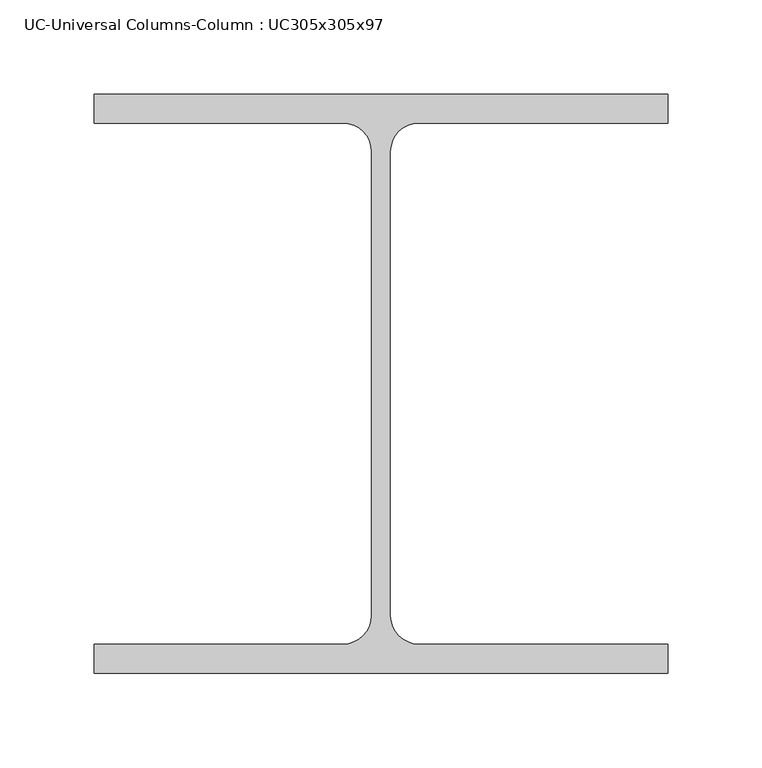
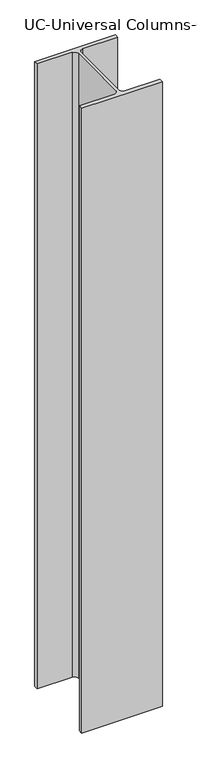
"""IFC4 building model written with IfcOpenShell, lengths in millimetres: column geometry, UC-Universal Columns-Column : UC305x305x97."""

from ifc_helpers import new_model, si_unit, point, frame, frame_2d, origin, place, context, project, spatial, polyline, circle_curve, trimmed, segment, composite_curve, outline, extrude, source, transform, mapped, element, save


def uc_universal_columns_column_uc305x305x97_2af35403(model_context):
    return source(origin(), model_context, "Body", "SweptSolid", [
        extrude(outline(composite_curve([segment(polyline([(152.65, 153.95), (152.65, 138.55), (20.15, 138.55)]), True, "CONTINUOUS"), segment(trimmed(circle_curve(frame_2d((20.15, 123.35)), 15.2), [point((20.15, 138.55))], [point((4.95, 123.35))], True, "CARTESIAN"), True, "CONTINUOUS"), segment(polyline([(4.95, 123.35), (4.95, -123.35)]), True, "CONTINUOUS"), segment(trimmed(circle_curve(frame_2d((20.15, -123.35)), 15.2), [point((4.95, -123.35))], [point((20.15, -138.55))], True, "CARTESIAN"), True, "CONTINUOUS"), segment(polyline([(20.15, -138.55), (152.65, -138.55), (152.65, -153.95), (-152.65, -153.95), (-152.65, -138.55), (-20.15, -138.55)]), True, "CONTINUOUS"), segment(trimmed(circle_curve(frame_2d((-20.15, -123.35)), 15.2), [point((-20.15, -138.55))], [point((-4.95, -123.35))], True, "CARTESIAN"), True, "CONTINUOUS"), segment(polyline([(-4.95, -123.35), (-4.95, 123.35)]), True, "CONTINUOUS"), segment(trimmed(circle_curve(frame_2d((-20.15, 123.35)), 15.2), [point((-4.95, 123.35))], [point((-20.15, 138.55))], True, "CARTESIAN"), True, "CONTINUOUS"), segment(polyline([(-20.15, 138.55), (-152.65, 138.55), (-152.65, 153.95), (152.65, 153.95)]), True, "CONTINUOUS")], self_intersect=False)), frame((0.0, 0.0, -2500.0), z_axis=(0.0, 0.0, 1.0), x_axis=(1.0, 0.0, 0.0)), (0.0, 0.0, 1.0), 2500.0),
    ])


if __name__ == "__main__":
    model = new_model("IFC4")
    model_context = context("Model", 3, world=origin())
    ifc_project = project(units=[si_unit("LENGTHUNIT", "METRE", prefix="MILLI")], contexts=[model_context])
    site = spatial("IfcSite", under=ifc_project)
    building = spatial("IfcBuilding", under=site)
    placement = place(None, origin())
    uc_universal_columns_column_uc305x305x97_shape = uc_universal_columns_column_uc305x305x97_2af35403(model_context)
    element("IfcColumn", 1, ObjectType="UC-Universal Columns-Column : UC305x305x97", at=placement, inside=building, context=model_context, shape_type="MappedRepresentation", body=[
        mapped(uc_universal_columns_column_uc305x305x97_shape, transform((0.0, 0.0, 0.0), x_axis=(1.0, 0.0, 0.0), y_axis=(0.0, 1.0, 0.0), z_axis=(0.0, 0.0, 1.0))),
    ])
    save(model, "model.ifc")

# Revit data of these elements
# Type "UC-Universal Columns-Column : UC305x305x97"
#   Section Name Key = "UC305x305x97"
#   Width = 30.53 cm
#   Web Thickness = 0.99 cm
#   Web Fillet = 1.52 cm
#   Warping Constant = 1560000.0 cm⁶
#   Torsional Moment of Inertia = 91.20 cm⁴
#   Section Area = 123.0 cm²
#   Plastic Modulus weak axis = 726.0 cm³
#   Plastic Modulus strong axis = 1592.0 cm³
#   Nominal Weight = 96.8996 kgf/m
#   Moment of Inertia weak axis = 7308.00 cm⁴
#   Moment of Inertia strong axis = 22249.00 cm⁴
#   Height = 30.79 cm
#   Flange Thickness = 1.54 cm
#   Elastic Modulus weak axis = 479.0 cm³
#   Elastic Modulus strong axis = 1445.0 cm³
#   Centroid Vertical = 15.395 cm
#   Centroid Horizontal = 15.265 cm
#   Bolt Spacing = 14.0 cm
#   Structural Material [instance default] = Metal - Steel 43-275
#   Type Comments = ""
#   Assembly Code = ""
# Element 1 (IfcColumn, "UC-Universal Columns-Column : UC305x305x97")
#   Materials on its faces: "Metal - Steel 43-275"
# Materials
#   "Metal - Steel 43-275": class "Metal", colour RGB 247 247 247, transparency 0, Cost = 0
